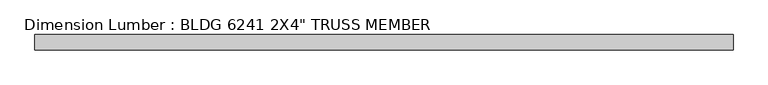
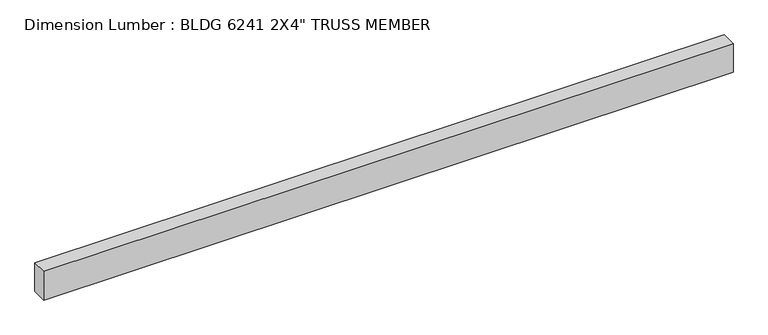
"""IFC4 building model written with IfcOpenShell, lengths in millimetres: beam geometry."""

from ifc_helpers import new_model, si_unit, frame, origin, place, context, project, spatial, polyline, outline, extrude, source, transform, mapped, element, save


def beam_71e3b4ab(model_context):
    return source(origin(), model_context, "Body", "SweptSolid", [
        extrude(outline(polyline([(1168.4, 25.4), (1168.4, -25.4), (-1143.0, -25.4), (-1143.0, 25.4), (1168.4, 25.4)])), frame((0.0, 0.0, -50.8), z_axis=(0.0, 0.0, 1.0), x_axis=(1.0, 0.0, 0.0)), (0.0, 0.0, 1.0), 101.6),
    ])


if __name__ == "__main__":
    model = new_model("IFC4")
    model_context = context("Model", 3, world=origin())
    ifc_project = project(units=[si_unit("LENGTHUNIT", "METRE", prefix="MILLI")], contexts=[model_context])
    site = spatial("IfcSite", under=ifc_project)
    building = spatial("IfcBuilding", under=site)
    placement = place(None, origin())
    beam_shape = beam_71e3b4ab(model_context)
    element("IfcBeam", 1, ObjectType="Dimension Lumber : BLDG 6241 2X4\" TRUSS MEMBER", at=placement, inside=building, context=model_context, shape_type="MappedRepresentation", body=[
        mapped(beam_shape, transform((0.0, 0.0, 0.0), x_axis=(1.0, 0.0, 0.0), y_axis=(0.0, 1.0, 0.0), z_axis=(0.0, 0.0, 1.0))),
    ])
    save(model, "model.ifc")

# Revit data of these elements
# Type "Dimension Lumber : BLDG 6241 2X4\" TRUSS MEMBER"
#   Assembly Code = "B10"
#   A = 0.273472 SF
#   Length [instance default] = 5' - 0"
#   b = 0' - 2"
#   d = 0' - 4"
#   Structural Material [instance default] = Softwood, Lumber
# Element 1 (IfcBeam, "Dimension Lumber : BLDG 6241 2X4\" TRUSS MEMBER")
#   Materials on its faces: "Softwood, Lumber"
# Materials
#   "Softwood, Lumber": class "Wood", colour RGB 223 192 134, transparency 0, Description = "Pinus Echinata", Cost = 0
